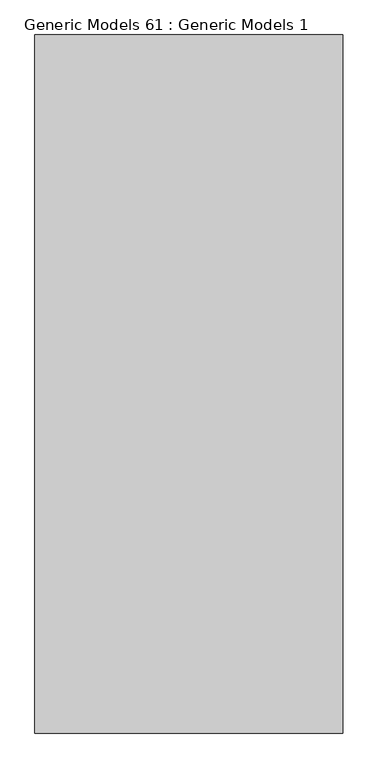
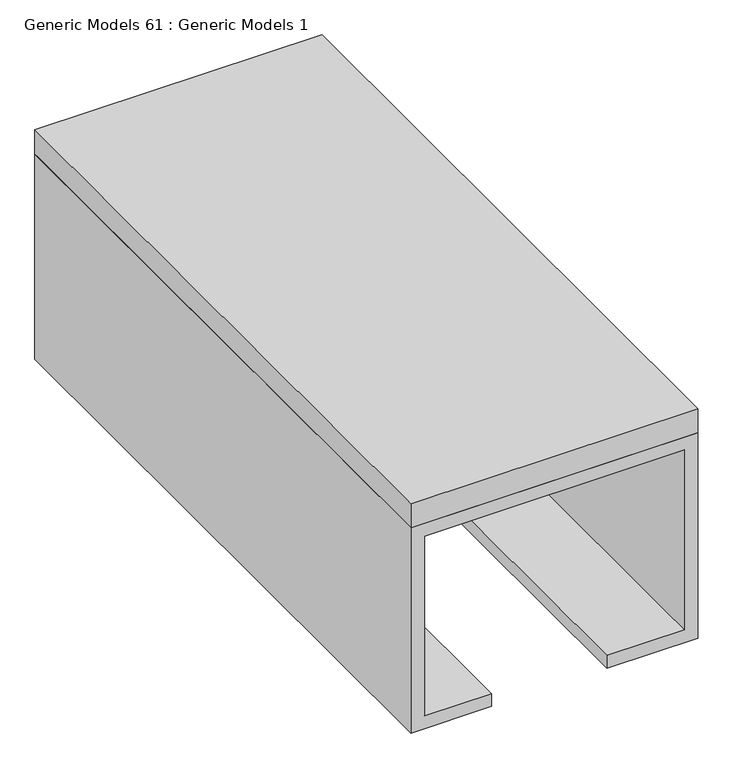
"""IFC4 building model written with IfcOpenShell, lengths in millimetres: proxy geometry, Generic Models 61 : Generic Models 1."""

from ifc_helpers import new_model, si_unit, frame, origin, place, context, project, spatial, polyline, outline, extrude, source, transform, mapped, element, save


def generic_models_61_generic_models_1_9775dfd0(model_context):
    return source(origin(), model_context, "Body", "SweptSolid", [
        extrude(outline(polyline([(51176.9547769, 0.0), (50639.5319345, 0.0), (50639.5319345, 1219.2), (51176.9547769, 1219.2), (51176.9547769, 0.0)])), frame((0.0, 0.0, 2410.0107871), z_axis=(0.0, 0.0, 1.0), x_axis=(1.0, 0.0, 0.0)), (0.0, 0.0, 1.0), 47.4392129),
        extrude(outline(polyline([(2028.825, 50664.9319345), (2384.425, 50664.9319345), (2384.425, 51151.5547769), (2028.825, 51151.5547769), (2028.825, 51006.375), (2003.425, 51006.375), (2003.425, 51176.9547769), (2409.825, 51176.9547769), (2409.825, 50639.5319345), (2003.425, 50639.5319345), (2003.425, 50790.475), (2028.825, 50790.475), (2028.825, 50664.9319345)])), frame((0.0, 0.0, 0.0), z_axis=(0.0, 1.0, 0.0), x_axis=(0.0, 0.0, 1.0)), (0.0, 0.0, 1.0), 1219.2),
    ])


if __name__ == "__main__":
    model = new_model("IFC4")
    model_context = context("Model", 3, world=origin())
    ifc_project = project(units=[si_unit("LENGTHUNIT", "METRE", prefix="MILLI")], contexts=[model_context])
    site = spatial("IfcSite", under=ifc_project)
    building = spatial("IfcBuilding", under=site)
    placement = place(None, origin())
    generic_models_61_generic_models_1_shape = generic_models_61_generic_models_1_9775dfd0(model_context)
    element("IfcBuildingElementProxy", 1, Name="Generic Models 61 : Generic Models 1", ObjectType="Generic Models 61 : Generic Models 1", at=placement, inside=building, context=model_context, shape_type="MappedRepresentation", body=[
        mapped(generic_models_61_generic_models_1_shape, transform((0.0, 0.0, 0.0), x_axis=(1.0, 0.0, 0.0), y_axis=(0.0, 1.0, 0.0), z_axis=(0.0, 0.0, 1.0))),
    ])
    save(model, "model.ifc")

# Revit data of these elements
# Element 1 (IfcBuildingElementProxy, "Generic Models 61 : Generic Models 1")
#   Materials on its faces: "ACOUSTICAL SOUND BARRIER"
# Materials
#   "ACOUSTICAL SOUND BARRIER": class "Generic", colour RGB 215 215 215, transparency 0, Cost = 0
